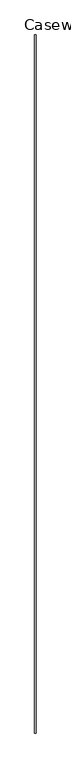
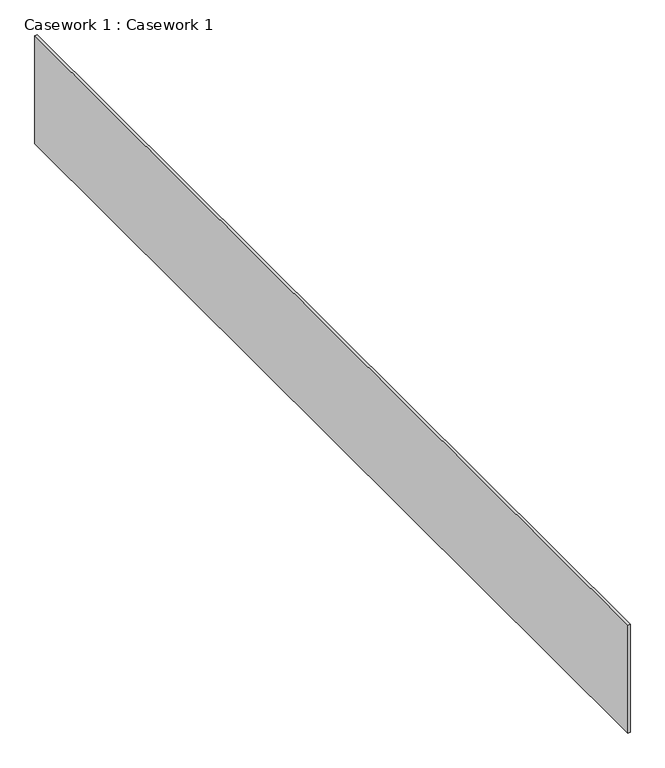
"""IFC4 building model written with IfcOpenShell, lengths in millimetres: furniture geometry, Casework 1 : Casework 1."""

from ifc_helpers import new_model, si_unit, frame, origin, place, context, project, spatial, polyline, outline, extrude, source, transform, mapped, element, save


def casework_1_casework_1_ae69b3e2(model_context):
    return source(origin(), model_context, "Body", "SweptSolid", [
        extrude(outline(polyline([(-38594.2176606, 259784.089454), (-38594.2176606, 248040.6639557), (-38619.6176606, 248040.6639557), (-38619.6176606, 259784.089454), (-38594.2176606, 259784.089454)])), frame((0.0, 0.0, 3340.1), z_axis=(0.0, 0.0, 1.0), x_axis=(1.0, 0.0, 0.0)), (0.0, 0.0, 1.0), 1303.445648),
    ])


if __name__ == "__main__":
    model = new_model("IFC4")
    model_context = context("Model", 3, world=origin())
    ifc_project = project(units=[si_unit("LENGTHUNIT", "METRE", prefix="MILLI")], contexts=[model_context])
    site = spatial("IfcSite", under=ifc_project)
    building = spatial("IfcBuilding", under=site)
    placement = place(None, origin())
    casework_1_casework_1_shape = casework_1_casework_1_ae69b3e2(model_context)
    element("IfcFurniture", 1, ObjectType="Casework 1 : Casework 1", at=placement, inside=building, context=model_context, shape_type="MappedRepresentation", body=[
        mapped(casework_1_casework_1_shape, transform((0.0, 0.0, 0.0), x_axis=(1.0, 0.0, 0.0), y_axis=(0.0, 1.0, 0.0), z_axis=(0.0, 0.0, 1.0))),
    ])
    save(model, "model.ifc")

# Revit data of these elements
# Element 1 (IfcFurniture, "Casework 1 : Casework 1")
#   Materials on its faces: "METAL PANEL (DARK BRONZE) - TO MATCH MAIN BUILDING ACCENT METAL"
# Materials
#   "METAL PANEL (DARK BRONZE) - TO MATCH MAIN BUILDING ACCENT METAL": class "Generic", colour RGB 88 62 61, transparency 0, Cost = 0
